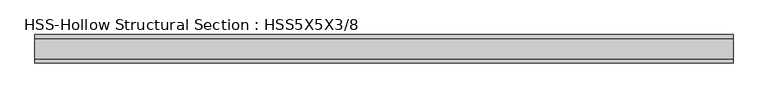
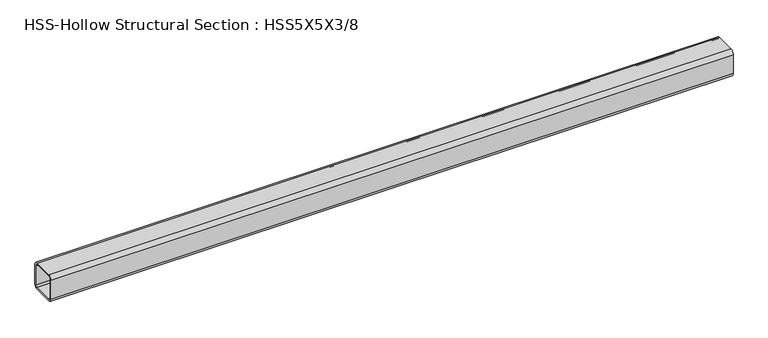
"""IFC4 building model written with IfcOpenShell, lengths in millimetres: member geometry, HSS-Hollow Structural Section : HSS5X5X3/8."""

from ifc_helpers import new_model, si_unit, point, frame, frame_2d, origin, place, context, project, spatial, polyline, circle_curve, trimmed, segment, composite_curve, outline, extrude, source, transform, mapped, element, save


def hss_hollow_structural_section_hss5x5x3_8_44fa9f29(model_context):
    return source(origin(), model_context, "Body", "SweptSolid", [
        extrude(outline(composite_curve([segment(polyline([(63.5, 45.7708), (63.5, -45.7708)]), True, "CONTINUOUS"), segment(trimmed(circle_curve(frame_2d((45.7708, -45.7708)), 17.7292), [point((63.5, -45.7708))], [point((45.7708, -63.5))], False, "CARTESIAN"), True, "CONTINUOUS"), segment(polyline([(45.7708, -63.5), (-45.7708, -63.5)]), True, "CONTINUOUS"), segment(trimmed(circle_curve(frame_2d((-45.7708, -45.7708)), 17.7292), [point((-45.7708, -63.5))], [point((-63.5, -45.7708))], False, "CARTESIAN"), True, "CONTINUOUS"), segment(polyline([(-63.5, -45.7708), (-63.5, 45.7708)]), True, "CONTINUOUS"), segment(trimmed(circle_curve(frame_2d((-45.7708, 45.7708)), 17.7292), [point((-63.5, 45.7708))], [point((-45.7708, 63.5))], False, "CARTESIAN"), True, "CONTINUOUS"), segment(polyline([(-45.7708, 63.5), (45.7708, 63.5)]), True, "CONTINUOUS"), segment(trimmed(circle_curve(frame_2d((45.7708, 45.7708)), 17.7292), [point((45.7708, 63.5))], [point((63.5, 45.7708))], False, "CARTESIAN"), True, "CONTINUOUS")], self_intersect=False), holes=[composite_curve([segment(trimmed(circle_curve(frame_2d((-45.7708, 45.7708)), 8.8646), [point((-45.7708, 54.6354))], [point((-54.6354, 45.7708))], True, "CARTESIAN"), True, "CONTINUOUS"), segment(polyline([(-54.6354, 45.7708), (-54.6354, -45.7708)]), True, "CONTINUOUS"), segment(trimmed(circle_curve(frame_2d((-45.7708, -45.7708)), 8.8646), [point((-54.6354, -45.7708))], [point((-45.7708, -54.6354))], True, "CARTESIAN"), True, "CONTINUOUS"), segment(polyline([(-45.7708, -54.6354), (45.7708, -54.6354)]), True, "CONTINUOUS"), segment(trimmed(circle_curve(frame_2d((45.7708, -45.7708)), 8.8646), [point((45.7708, -54.6354))], [point((54.6354, -45.7708))], True, "CARTESIAN"), True, "CONTINUOUS"), segment(polyline([(54.6354, -45.7708), (54.6354, 45.7708)]), True, "CONTINUOUS"), segment(trimmed(circle_curve(frame_2d((45.7708, 45.7708)), 8.8646), [point((54.6354, 45.7708))], [point((45.7708, 54.6354))], True, "CARTESIAN"), True, "CONTINUOUS"), segment(polyline([(45.7708, 54.6354), (-45.7708, 54.6354)]), True, "CONTINUOUS")], self_intersect=False)]), frame((-1575.036148, 0.0, 0.0), z_axis=(1.0, 0.0, 0.0), x_axis=(0.0, 1.0, 0.0)), (0.0, 0.0, 1.0), 3114.5436004),
    ])


if __name__ == "__main__":
    model = new_model("IFC4")
    model_context = context("Model", 3, world=origin())
    ifc_project = project(units=[si_unit("LENGTHUNIT", "METRE", prefix="MILLI")], contexts=[model_context])
    site = spatial("IfcSite", under=ifc_project)
    building = spatial("IfcBuilding", under=site)
    placement = place(None, origin())
    hss_hollow_structural_section_hss5x5x3_8_shape = hss_hollow_structural_section_hss5x5x3_8_44fa9f29(model_context)
    element("IfcMember", 1, ObjectType="HSS-Hollow Structural Section : HSS5X5X3/8", at=placement, inside=building, context=model_context, shape_type="MappedRepresentation", body=[
        mapped(hss_hollow_structural_section_hss5x5x3_8_shape, transform((0.0, 0.0, 0.0), x_axis=(1.0, 0.0, 0.0), y_axis=(0.0, 1.0, 0.0), z_axis=(0.0, 0.0, 1.0))),
    ])
    save(model, "model.ifc")

# Revit data of these elements
# Type "HSS-Hollow Structural Section : HSS5X5X3/8"
#   Assembly Code = "B10"
#   Shape = "Square"
#   W = 22.3
#   Ht = 0' - 5"
#   Length [instance default] = 5' - 0"
#   b = 0' - 5"
#   kr = 0' - 0.698"
#   t = 0' - 0.349"
#   A = 0.0429167 SF
#   Structural Material [instance default] = Steel ASTM A500, Grade B, Rectangular and Square
# Element 1 (IfcMember, "HSS-Hollow Structural Section : HSS5X5X3/8")
#   Materials on its faces: "Steel ASTM A500, Grade B, Rectangular and Square"
# Materials
#   "Steel ASTM A500, Grade B, Rectangular and Square": class "Metal", colour RGB 199 199 199, transparency 0, Description = "Carbon steel", Cost = 0
